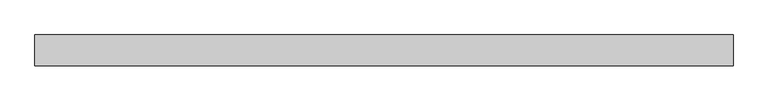
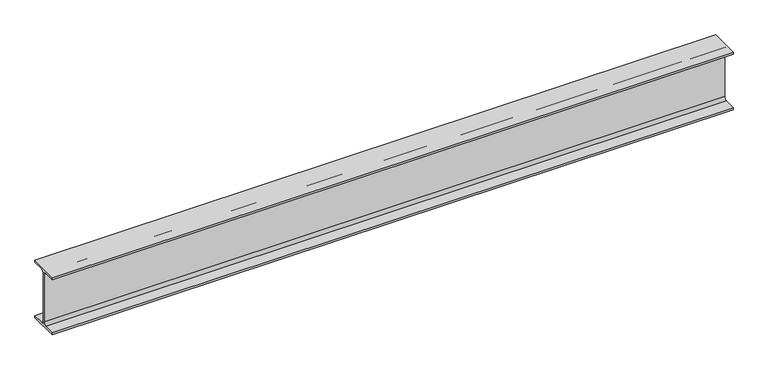
"""IFC4 building model written with IfcOpenShell, lengths in millimetres: beam geometry, 0912_Steel Framing_H-KSD3502 : H_SB_ASB_H-250x125x6x9."""

from ifc_helpers import new_model, si_unit, point, frame, frame_2d, origin, place, context, project, spatial, polyline, circle_curve, trimmed, segment, composite_curve, outline, extrude, source, transform, mapped, element, save


def beam_7d78cf47(model_context):
    return source(origin(), model_context, "Body", "SweptSolid", [
        extrude(outline(composite_curve([segment(polyline([(62.5, -116.0), (62.5, -125.0), (-62.5, -125.0), (-62.5, -116.0), (-15.0, -116.0)]), True, "CONTINUOUS"), segment(trimmed(circle_curve(frame_2d((-15.0, -104.0)), 12.0), [point((-15.0, -116.0))], [point((-3.0, -104.0))], True, "CARTESIAN"), True, "CONTINUOUS"), segment(polyline([(-3.0, -104.0), (-3.0, 104.0)]), True, "CONTINUOUS"), segment(trimmed(circle_curve(frame_2d((-15.0, 104.0)), 12.0), [point((-3.0, 104.0))], [point((-15.0, 116.0))], True, "CARTESIAN"), True, "CONTINUOUS"), segment(polyline([(-15.0, 116.0), (-62.5, 116.0), (-62.5, 125.0), (62.5, 125.0), (62.5, 116.0), (15.0, 116.0)]), True, "CONTINUOUS"), segment(trimmed(circle_curve(frame_2d((15.0, 104.0)), 12.0), [point((15.0, 116.0))], [point((3.0, 104.0))], True, "CARTESIAN"), True, "CONTINUOUS"), segment(polyline([(3.0, 104.0), (3.0, -104.0)]), True, "CONTINUOUS"), segment(trimmed(circle_curve(frame_2d((15.0, -104.0)), 12.0), [point((3.0, -104.0))], [point((15.0, -116.0))], True, "CARTESIAN"), True, "CONTINUOUS"), segment(polyline([(15.0, -116.0), (62.5, -116.0)]), True, "CONTINUOUS")], self_intersect=False)), frame((-1404.7192363, 0.0, 0.0), z_axis=(1.0, 0.0, 0.0), x_axis=(0.0, 1.0, 0.0)), (0.0, 0.0, 1.0), 2809.5192866),
    ])


if __name__ == "__main__":
    model = new_model("IFC4")
    model_context = context("Model", 3, world=origin())
    ifc_project = project(units=[si_unit("LENGTHUNIT", "METRE", prefix="MILLI")], contexts=[model_context])
    site = spatial("IfcSite", under=ifc_project)
    building = spatial("IfcBuilding", under=site)
    placement = place(None, origin())
    beam_shape = beam_7d78cf47(model_context)
    element("IfcBeam", 1, ObjectType="0912_Steel Framing_H-KSD3502 : H_SB_ASB_H-250x125x6x9", at=placement, inside=building, context=model_context, shape_type="MappedRepresentation", body=[
        mapped(beam_shape, transform((0.0, 0.0, 0.0), x_axis=(1.0, 0.0, 0.0), y_axis=(0.0, 1.0, 0.0), z_axis=(0.0, 0.0, 1.0))),
    ])
    save(model, "model.ifc")

# Revit data of these elements
# Type "0912_Steel Framing_H-KSD3502 : H_SB_ASB_H-250x125x6x9"
#   H_WM Code_1 = "S01AA003-00001 | Main Steel Structure Fabrication Work | Shelter/Building | Light Steel - Standard (30KG/M>Weight) | Material: (   )"
#   H_WM Code_2 = "S03AA029-00001 | Main Steel Structure Erection Work | Shelter/Building | Light Steel (30KG/M>Weight) | Material: (   )"
#   H_WM Code_3 = "S01AA010-00001 | Main Steel Structure Fabrication Work | Shelter/Building | Steel Painting/Coating | for Non-Fireproofed Steel Surface, Surface Preparation, Primer, Second & Final Coat | Material: (   )"
#   H_Q'ty Cal Type Tag = "SB-Q2"
#   Width = 12.5 cm
#   Web Thickness = 0.6 cm
#   Web Fillet = 1.2 cm
#   Warping Constant = 42539.8 cm⁶
#   W = 0
#   Torsional Moment of Inertia = 7.8102 cm⁴
#   Section Area = 37.66 cm²
#   Plastic Modulus weak axis = 73.1 cm³
#   Plastic Modulus strong axis = 366.0 cm³
#   Perimeter = 0.97 m²/m
#   Nominal Weight = 29.60 kgf/m
#   Moment of Inertia weak axis = 294.00 cm⁴
#   Moment of Inertia strong axis = 4050.00 cm⁴
#   Height = 25.0 cm
#   Flange Thickness = 0.9 cm
#   Elastic Modulus weak axis = 47.0 cm³
#   Elastic Modulus strong axis = 324.0 cm³
#   Centroid Vertical = 12.5 cm
#   Centroid Horizontal = 6.25 cm
#   Ix = 40500000
#   Length [instance default] = 1.5240 m
#   Zx = 366000
#   b = 0.1250 m
#   h = 0.2500 m
#   r = 0.0120 m
#   s = 0.0060 m
#   t = 0.0090 m
#   A = 0.003766 m²
#   Structural Material [instance default] = Steel, 45-345
#   Assembly Code = ""
# Element 1 (IfcBeam, "0912_Steel Framing_H-KSD3502 : H_SB_ASB_H-250x125x6x9")
#   Structural Material = none
# Materials
#   "Steel, 45-345": class "Metal", colour RGB 189 187 185, transparency 0, Description = "Steel 345 MPa", Cost = 0
